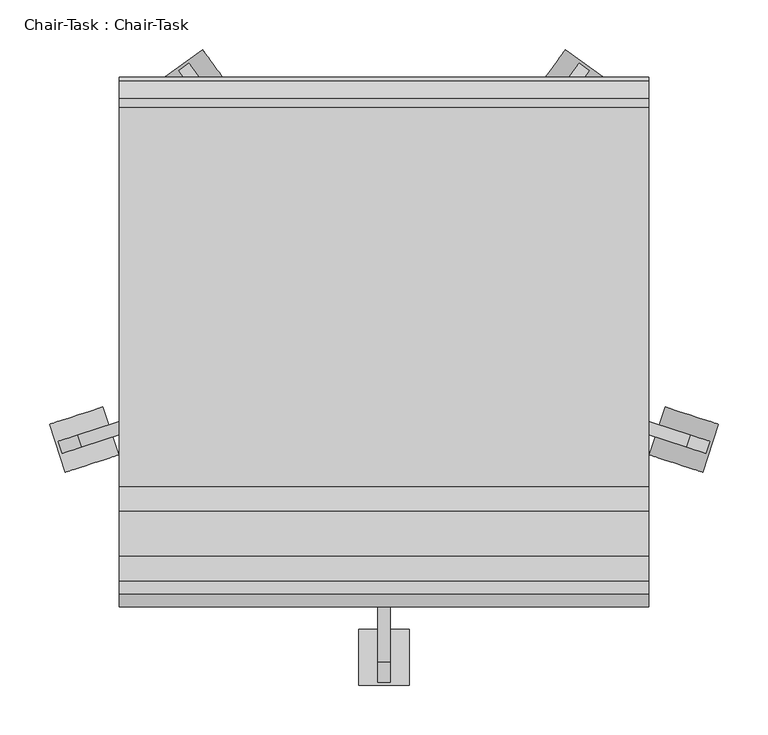
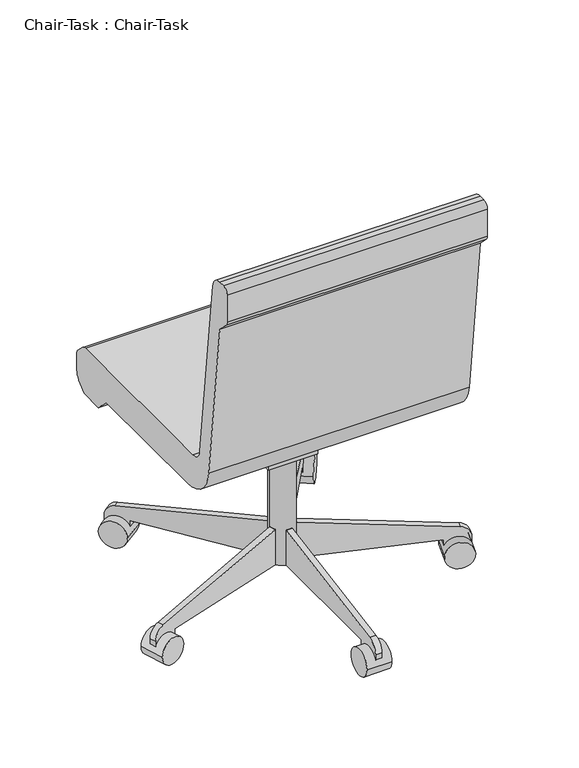
"""IFC4 building model written with IfcOpenShell, lengths in millimetres: furniture geometry, Chair-Task : Chair-Task."""

import ifcopenshell
import ifcopenshell.guid

model = None  # the IFC model being written
_history = None  # IfcOwnerHistory: only IFC2X3 demands one
_inside = {}  # id of a spatial element -> (the spatial element, [elements in it])
_under = {}  # id of a project, library or spatial element -> (it, [spatial elements below it])
_declared = {}  # id of a project -> (the project, [libraries it declares])
_typed = {}  # id of a type object -> (the type object, [elements of that type])
_made_of = {}  # id of a material, layer set ... -> (it, [elements and type objects made of it])


def new_model(schema):
    """Start an empty IFC model of exactly this schema.

    Asked for "IFC4X3", IfcOpenShell would pick the latest addendum, in which some entities
    have other attributes; the version numbers below select the first issue.
    IFC2X3 requires an IfcOwnerHistory on every rooted entity: one is made here for all.
    """
    global model, _history
    if schema == "IFC4X3":
        model = ifcopenshell.file(schema_version=(4, 3, 0, 0))
    else:
        model = ifcopenshell.file(schema=schema)
    _inside.clear()
    _under.clear()
    _declared.clear()
    _typed.clear()
    _made_of.clear()
    _history = None
    if model.schema == "IFC2X3":
        org = make("IfcOrganization", Name="unknown")
        user = make(
            "IfcPersonAndOrganization",
            ThePerson=make("IfcPerson", FamilyName="unknown"),
            TheOrganization=org,
        )
        app = make(
            "IfcApplication",
            ApplicationDeveloper=org,
            Version="unknown",
            ApplicationFullName="unknown",
            ApplicationIdentifier="unknown",
        )
        _history = make(
            "IfcOwnerHistory",
            OwningUser=user,
            OwningApplication=app,
            ChangeAction="ADDED",
            CreationDate=0,
        )
    return model


def make(cls, **values):
    """One entity of the class cls with the attributes given. An attribute that is None is left unset."""
    return model.create_entity(
        cls, **{name: value for name, value in values.items() if value is not None}
    )


def rooted(cls, **values):
    """An entity with a GlobalId (a new one), such as an element, a storey or a relation."""
    return make(cls, GlobalId=ifcopenshell.guid.new(), OwnerHistory=_history, **values)


def si_unit(unit_type, name, prefix=None):
    """IfcSIUnit, for example si_unit("LENGTHUNIT", "METRE", prefix="MILLI")."""
    return make("IfcSIUnit", UnitType=unit_type, Prefix=prefix, Name=name)


def assignment(units):
    """IfcUnitAssignment: the units of a project."""
    return None if units is None else make("IfcUnitAssignment", Units=units)


def point(xyz):
    """IfcCartesianPoint."""
    return None if xyz is None else make("IfcCartesianPoint", Coordinates=xyz)


def direction(xyz):
    """IfcDirection."""
    return None if xyz is None else make("IfcDirection", DirectionRatios=xyz)


def frame(location, z_axis=None, x_axis=None):
    """IfcAxis2Placement3D, a coordinate frame: its origin and axes. An axis left out is left unset."""
    return make(
        "IfcAxis2Placement3D",
        Location=point(location),
        Axis=direction(z_axis),
        RefDirection=direction(x_axis),
    )


def frame_2d(location, x_axis=None):
    """IfcAxis2Placement2D, a coordinate frame in the plane: its origin and x axis."""
    return make(
        "IfcAxis2Placement2D", Location=point(location), RefDirection=direction(x_axis)
    )


def origin():
    """The frame at (0, 0, 0) with its axes left unset."""
    return frame((0.0, 0.0, 0.0))


def place(relative_to, where):
    """IfcLocalPlacement: puts the frame where relative to a parent placement (None: the world)."""
    return make(
        "IfcLocalPlacement", PlacementRelTo=relative_to, RelativePlacement=where
    )


def context(
    kind, dimensions, precision=None, world=None, true_north=None, identifier=None
):
    """IfcGeometricRepresentationContext, for example the 3D "Model" context."""
    return make(
        "IfcGeometricRepresentationContext",
        ContextIdentifier=identifier,
        ContextType=kind,
        CoordinateSpaceDimension=dimensions,
        Precision=precision,
        WorldCoordinateSystem=world,
        TrueNorth=true_north,
    )


def project(units=None, contexts=None):
    """IfcProject with its units and contexts."""
    return rooted(
        "IfcProject",
        Name="project",
        RepresentationContexts=contexts,
        UnitsInContext=assignment(units),
    )


def spatial(cls, under=None, at=None, **own):
    """A site, building, storey or space (cls), placed at a placement, below another one or the project."""
    s = rooted(cls, ObjectPlacement=at, **own)
    if under is not None:
        _under.setdefault(under.id(), (under, []))[1].append(s)
    return s


def polyline(points):
    """IfcPolyline through the points."""
    return make("IfcPolyline", Points=[point(p) for p in points])


def circle_curve(where, radius):
    """IfcCircle in the frame where."""
    return make("IfcCircle", Position=where, Radius=radius)


def trimmed(basis, trim1, trim2, sense, master):
    """IfcTrimmedCurve: the piece of a basis curve between two trims."""
    return make(
        "IfcTrimmedCurve",
        BasisCurve=basis,
        Trim1=trim1,
        Trim2=trim2,
        SenseAgreement=sense,
        MasterRepresentation=master,
    )


def segment(curve, same_sense, transition):
    """IfcCompositeCurveSegment."""
    return make(
        "IfcCompositeCurveSegment",
        Transition=transition,
        SameSense=same_sense,
        ParentCurve=curve,
    )


def composite_curve(segments, self_intersect=None):
    """IfcCompositeCurve: segments joined end to end."""
    return make("IfcCompositeCurve", Segments=segments, SelfIntersect=self_intersect)


def outline(outer, holes=None, kind="AREA"):
    """IfcArbitraryClosedProfileDef: a profile drawn as a closed curve; with holes, ...WithVoids."""
    if holes is None:
        return make("IfcArbitraryClosedProfileDef", ProfileType=kind, OuterCurve=outer)
    return make(
        "IfcArbitraryProfileDefWithVoids",
        ProfileType=kind,
        OuterCurve=outer,
        InnerCurves=holes,
    )


def extrude(swept, where, along, depth):
    """IfcExtrudedAreaSolid: the profile swept, set in the frame where, extruded along a direction by depth."""
    return make(
        "IfcExtrudedAreaSolid",
        SweptArea=swept,
        Position=where,
        ExtrudedDirection=direction(along),
        Depth=depth,
    )


def shape(context_of_items, identifier, shape_type, items):
    """IfcShapeRepresentation: the items that make up one representation, for example the "Body"."""
    return make(
        "IfcShapeRepresentation",
        ContextOfItems=context_of_items,
        RepresentationIdentifier=identifier,
        RepresentationType=shape_type,
        Items=items,
    )


def source(mapping_origin, context_of_items, identifier, shape_type, items):
    """IfcRepresentationMap: a shape defined once, which mapped items show again and again."""
    return make(
        "IfcRepresentationMap",
        MappingOrigin=mapping_origin,
        MappedRepresentation=shape(context_of_items, identifier, shape_type, items),
    )


def transform(
    local_origin,
    x_axis=None,
    y_axis=None,
    z_axis=None,
    scale=None,
    scale2=None,
    scale3=None,
    uniform=True,
):
    """IfcCartesianTransformationOperator3D, or its non-uniform kind. x_axis, y_axis, z_axis: its Axis1, 2, 3."""
    if uniform:
        return make(
            "IfcCartesianTransformationOperator3D",
            Axis1=direction(x_axis),
            Axis2=direction(y_axis),
            LocalOrigin=point(local_origin),
            Scale=scale,
            Axis3=direction(z_axis),
        )
    return make(
        "IfcCartesianTransformationOperator3DnonUniform",
        Axis1=direction(x_axis),
        Axis2=direction(y_axis),
        LocalOrigin=point(local_origin),
        Scale=scale,
        Axis3=direction(z_axis),
        Scale2=scale2,
        Scale3=scale3,
    )


def mapped(mapping_source, mapping_target):
    """IfcMappedItem: shows the shape of a source again, moved by a transform."""
    return make(
        "IfcMappedItem", MappingSource=mapping_source, MappingTarget=mapping_target
    )


def made_of(thing, what):
    """Note that an element or type object is made of a material, layer set ...; save() writes the relation."""
    if what is not None:
        _made_of.setdefault(what.id(), (what, []))[1].append(thing)
    return thing


def element(
    cls,
    number,
    at=None,
    inside=None,
    cuts=None,
    type_object=None,
    material=None,
    context=None,
    identifier="Body",
    shape_type=None,
    held_by="IfcProductDefinitionShape",
    body=None,
    shapes=None,
    **own,
):
    """One element of the class cls, such as IfcWall. Its Tag is "e" and its number.

    at: its placement. inside: the storey or other place that contains it. cuts: it is an
    opening in that element (IfcRelVoidsElement). A single representation is given by context,
    identifier, shape_type and body (its items); several are given by shapes. held_by: the class
    of the entity that holds the representations. save() writes the other relations.
    """
    e = rooted(cls, Tag="e%d" % number, ObjectPlacement=at, **own)
    if body is not None:
        shapes = [shape(context, identifier, shape_type, body)]
    if shapes is not None:
        e.Representation = make(held_by, Representations=shapes)
    if inside is not None:
        _inside.setdefault(inside.id(), (inside, []))[1].append(e)
    if cuts is not None:
        rooted(
            "IfcRelVoidsElement", RelatingBuildingElement=cuts, RelatedOpeningElement=e
        )
    if type_object is not None:
        _typed.setdefault(type_object.id(), (type_object, []))[1].append(e)
    return made_of(e, material)


def aggregate(whole, parts):
    """IfcRelAggregates: a whole, such as a stair, and the parts it consists of."""
    return rooted("IfcRelAggregates", RelatingObject=whole, RelatedObjects=parts)


def save(model, path):
    """Write the relations noted so far, then the file.

    IfcRelAggregates (storeys below a building ...), IfcRelContainedInSpatialStructure (elements
    in a storey), IfcRelDefinesByType, IfcRelAssociatesMaterial and IfcRelDeclares: one each for
    every whole, place, type object, material and project.
    """
    for whole, parts in _under.values():
        aggregate(whole, parts)
    for where, things in _inside.values():
        rooted(
            "IfcRelContainedInSpatialStructure",
            RelatedElements=things,
            RelatingStructure=where,
        )
    for kind, things in _typed.values():
        rooted("IfcRelDefinesByType", RelatedObjects=things, RelatingType=kind)
    for what, things in _made_of.values():
        rooted("IfcRelAssociatesMaterial", RelatedObjects=things, RelatingMaterial=what)
    for by, libraries in _declared.values():
        rooted("IfcRelDeclares", RelatingContext=by, RelatedDefinitions=libraries)
    model.write(path)


def chair_task_chair_task_e9ee4668(model_context):
    return source(origin(), model_context, "Body", "SweptSolid", [
        extrude(outline(composite_curve([segment(trimmed(circle_curve(frame_2d((0.0, -28.2002728)), 28.2002727), [point((0.0, -56.4005455))], [point((0.0, 0.0))], False, "CARTESIAN"), True, "CONTINUOUS"), segment(trimmed(circle_curve(frame_2d((0.0, -28.2002728)), 28.2002727), [point((0.0, 0.0))], [point((0.0, -56.4005455))], False, "CARTESIAN"), True, "CONTINUOUS")], self_intersect=False)), frame((461.9222851, -112.0381931, 28.1835944), z_axis=(0.30901699437494234, 0.9510565162951552, 0.0), x_axis=(0.0, 0.0, 1.0)), (0.0, 0.0, 1.0), 50.8),
        extrude(outline(composite_curve([segment(polyline([(292.1, 0.0), (292.1, 25.4), (342.9, 25.4), (342.9, 1.096947)]), True, "CONTINUOUS"), segment(trimmed(circle_curve(frame_2d((317.5, 1.096947)), 25.4), [point((342.9, 1.096947))], [point((321.9106636, -23.9171699))], False, "CARTESIAN"), True, "CONTINUOUS"), segment(polyline([(321.9106636, -23.9171699), (25.4, -76.2), (0.0, -76.2), (0.0, 0.0), (292.1, 0.0)]), True, "CONTINUOUS")], self_intersect=False)), frame((139.0285618, 12.9066928, 53.5835944), z_axis=(0.30901699437494234, 0.9510565162951552, 0.0), x_axis=(0.9510565162951552, -0.30901699437494234, 0.0)), (0.0, 0.0, 1.0), 12.7),
        extrude(outline(composite_curve([segment(trimmed(circle_curve(frame_2d((0.0, -28.2002727)), 28.2002727), [point((0.0, -56.4005454))], [point((0.0, 0.0))], False, "CARTESIAN"), True, "CONTINUOUS"), segment(trimmed(circle_curve(frame_2d((0.0, -28.2002727)), 28.2002727), [point((0.0, 0.0))], [point((0.0, -56.4005454))], False, "CARTESIAN"), True, "CONTINUOUS")], self_intersect=False)), frame((364.7373733, 283.6935518, 28.1835944), z_axis=(-0.8090169943749497, 0.58778525229247, 0.0), x_axis=(0.0, 0.0, 1.0)), (0.0, 0.0, 1.0), 50.8),
        extrude(outline(composite_curve([segment(polyline([(292.1, 0.0), (292.1, 25.4), (342.9, 25.4), (342.9, 1.096947)]), True, "CONTINUOUS"), segment(trimmed(circle_curve(frame_2d((317.5, 1.096947)), 25.4), [point((342.9, 1.096947))], [point((321.9106637, -23.9171699))], False, "CARTESIAN"), True, "CONTINUOUS"), segment(polyline([(321.9106637, -23.9171699), (25.3999999, -76.2), (0.0, -76.2), (0.0, 0.0), (292.1, 0.0)]), True, "CONTINUOUS")], self_intersect=False)), frame((146.1280776, 15.2134653, 53.5835944), z_axis=(-0.8090169943749498, 0.58778525229247, 0.0), x_axis=(0.58778525229247, 0.8090169943749498, 0.0)), (0.0, 0.0, 1.0), 12.7),
        extrude(outline(composite_curve([segment(trimmed(circle_curve(frame_2d((0.0, -28.2002727)), 28.2002727), [point((0.0, -56.4005454))], [point((0.0, 0.0))], False, "CARTESIAN"), True, "CONTINUOUS"), segment(trimmed(circle_curve(frame_2d((0.0, -28.2002727)), 28.2002727), [point((0.0, 0.0))], [point((0.0, -56.4005454))], False, "CARTESIAN"), True, "CONTINUOUS")], self_intersect=False)), frame((-82.755734, 283.6935518, 28.1835944), z_axis=(0.8090169943749459, 0.5877852522924751, 0.0), x_axis=(0.0, 0.0, -1.0)), (0.0, 0.0, 1.0), 50.8),
        extrude(outline(composite_curve([segment(polyline([(-292.1, 0.0), (0.0, 0.0), (0.0, -76.2), (-25.4, -76.2), (-321.9106637, -23.9171699)]), True, "CONTINUOUS"), segment(trimmed(circle_curve(frame_2d((-317.5, 1.096947)), 25.4), [point((-321.9106637, -23.9171699))], [point((-342.9000001, 1.096947))], False, "CARTESIAN"), True, "CONTINUOUS"), segment(polyline([(-342.9000001, 1.096947), (-342.9000001, 25.4), (-292.1, 25.4), (-292.1, 0.0)]), True, "CONTINUOUS")], self_intersect=False)), frame((135.8535618, 15.2134653, 53.5835944), z_axis=(0.8090169943749459, 0.5877852522924752, 0.0), x_axis=(0.5877852522924752, -0.8090169943749459, 0.0)), (0.0, 0.0, 1.0), 12.7),
        extrude(outline(composite_curve([segment(trimmed(circle_curve(frame_2d((0.0, -28.2002727)), 28.2002727), [point((0.0, -56.4005454))], [point((0.0, 0.0))], False, "CARTESIAN"), True, "CONTINUOUS"), segment(trimmed(circle_curve(frame_2d((0.0, -28.2002727)), 28.2002727), [point((0.0, 0.0))], [point((0.0, -56.4005454))], False, "CARTESIAN"), True, "CONTINUOUS")], self_intersect=False)), frame((-179.9406457, -112.0381931, 28.1835944), z_axis=(-0.30901699437494856, 0.9510565162951532, 0.0), x_axis=(0.0, 0.0, -1.0)), (0.0, 0.0, 1.0), 50.8),
        extrude(outline(composite_curve([segment(polyline([(-292.1, 0.0), (0.0, 0.0), (0.0, -76.2), (-25.4, -76.2), (-321.9106637, -23.9171699)]), True, "CONTINUOUS"), segment(trimmed(circle_curve(frame_2d((-317.5, 1.096947)), 25.4), [point((-321.9106637, -23.9171699))], [point((-342.9000001, 1.096947))], False, "CARTESIAN"), True, "CONTINUOUS"), segment(polyline([(-342.9000001, 1.096947), (-342.9000001, 25.4), (-292.1, 25.4), (-292.1, 0.0)]), True, "CONTINUOUS")], self_intersect=False)), frame((142.9530776, 12.9066928, 53.5835944), z_axis=(-0.30901699437494856, 0.9510565162951532, 0.0), x_axis=(0.9510565162951532, 0.30901699437494856, 0.0)), (0.0, 0.0, 1.0), 12.7),
        extrude(outline(composite_curve([segment(trimmed(circle_curve(frame_2d((-298.5540984, 28.1835944)), 28.2002727), [point((-270.3538256, 28.1835944))], [point((-326.7543711, 28.1835944))], False, "CARTESIAN"), True, "CONTINUOUS"), segment(trimmed(circle_curve(frame_2d((-298.5540984, 28.1835944)), 28.2002727), [point((-326.7543711, 28.1835944))], [point((-270.3538256, 28.1835944))], False, "CARTESIAN"), True, "CONTINUOUS")], self_intersect=False)), frame((115.5908197, 0.0, 0.0), z_axis=(1.0, 0.0, 0.0), x_axis=(0.0, 1.0, 0.0)), (0.0, 0.0, 1.0), 50.8),
        extrude(outline(composite_curve([segment(polyline([(-273.1540984, 53.5835944), (-273.1540984, 28.1835944), (-323.9540984, 28.1835944), (-323.9540984, 52.4866474)]), True, "CONTINUOUS"), segment(trimmed(circle_curve(frame_2d((-298.5540984, 52.4866474)), 25.4), [point((-323.9540984, 52.4866474))], [point((-302.9647621, 77.5007643))], False, "CARTESIAN"), True, "CONTINUOUS"), segment(polyline([(-302.9647621, 77.5007643), (-6.4540984, 129.7835944), (18.9459016, 129.7835944), (18.9459016, 53.5835944), (-273.1540984, 53.5835944)]), True, "CONTINUOUS")], self_intersect=False)), frame((134.6408197, 0.0, 0.0), z_axis=(1.0, 0.0, 0.0), x_axis=(0.0, 1.0, 0.0)), (0.0, 0.0, 1.0), 12.7),
        extrude(outline(composite_curve([segment(trimmed(circle_curve(frame_2d((140.9908197, 18.9459016)), 25.4), [point((115.5908197, 18.9459016))], [point((166.3908197, 18.9459016))], False, "CARTESIAN"), True, "CONTINUOUS"), segment(trimmed(circle_curve(frame_2d((140.9908197, 18.9459016)), 25.4), [point((166.3908197, 18.9459016))], [point((115.5908197, 18.9459016))], False, "CARTESIAN"), True, "CONTINUOUS")], self_intersect=False)), frame((0.0, 0.0, 53.5835944), z_axis=(0.0, 0.0, 1.0), x_axis=(1.0, 0.0, 0.0)), (0.0, 0.0, 1.0), 330.5914056),
        extrude(outline(polyline([(69.7459016, 383.7835944), (69.7459016, 371.0835944), (18.9459016, 283.0954134), (-19.1540984, 283.0954134), (-19.1540984, 383.7835944), (69.7459016, 383.7835944)])), frame((90.1908197, 0.0, 0.0), z_axis=(1.0, 0.0, 0.0), x_axis=(0.0, 1.0, 0.0)), (0.0, 0.0, 1.0), 101.6),
        extrude(outline(composite_curve([segment(polyline([(-126.2050455, 457.2), (255.0102301, 457.2)]), True, "CONTINUOUS"), segment(trimmed(circle_curve(frame_2d((255.0102301, 444.5)), 12.7), [point((255.0102301, 457.2))], [point((263.9604301, 453.510212))], False, "CARTESIAN"), True, "CONTINUOUS"), segment(polyline([(263.9604301, 453.510212), (281.8961016, 435.6939999)]), True, "CONTINUOUS"), segment(trimmed(circle_curve(frame_2d((272.9459016, 426.6837879)), 12.7), [point((281.8961016, 435.6939999))], [point((285.6459016, 426.6837879))], False, "CARTESIAN"), True, "CONTINUOUS"), segment(polyline([(285.6459016, 426.6837879), (285.6459016, 391.6405184)]), True, "CONTINUOUS"), segment(trimmed(circle_curve(frame_2d((260.2459016, 391.6405184)), 25.4), [point((285.6459016, 391.6405184))], [point((278.2663256, 373.7401184))], False, "CARTESIAN"), True, "CONTINUOUS"), segment(polyline([(278.2663256, 373.7401184), (260.2470284, 355.6), (209.4470284, 355.6), (181.0744602, 383.7835944), (-107.1089978, 383.7835944)]), True, "CONTINUOUS"), segment(trimmed(circle_curve(frame_2d((-107.1089978, 459.9835944)), 76.2), [point((-107.1089978, 383.7835944))], [point((-182.7870738, 451.0802913))], False, "CARTESIAN"), True, "CONTINUOUS"), segment(polyline([(-182.7870738, 451.0802913), (-222.3540984, 787.4), (-244.0343545, 809.0802561)]), True, "CONTINUOUS"), segment(trimmed(circle_curve(frame_2d((-235.0540984, 818.0605122)), 12.7), [point((-244.0343545, 809.0802561))], [point((-247.7540984, 818.0605122))], False, "CARTESIAN"), True, "CONTINUOUS"), segment(polyline([(-247.7540984, 818.0605122), (-247.7540984, 876.3)]), True, "CONTINUOUS"), segment(trimmed(circle_curve(frame_2d((-235.0540984, 876.3)), 12.7), [point((-247.7540984, 876.3))], [point((-235.0540984, 889.0))], False, "CARTESIAN"), True, "CONTINUOUS"), segment(polyline([(-235.0540984, 889.0), (-222.1789239, 889.0)]), True, "CONTINUOUS"), segment(trimmed(circle_curve(frame_2d((-222.1789239, 863.6)), 25.4), [point((-222.1789239, 889.0))], [point((-196.9528985, 866.5677677))], False, "CARTESIAN"), True, "CONTINUOUS"), segment(polyline([(-196.9528985, 866.5677677), (-151.4310708, 479.6322323)]), True, "CONTINUOUS"), segment(trimmed(circle_curve(frame_2d((-126.2050455, 482.6)), 25.4), [point((-151.4310708, 479.6322323))], [point((-126.2050455, 457.2))], True, "CARTESIAN"), True, "CONTINUOUS")], self_intersect=False)), frame((-125.7091803, 0.0, 0.0), z_axis=(1.0, 0.0, 0.0), x_axis=(0.0, 1.0, 0.0)), (0.0, 0.0, 1.0), 533.4),
    ])


if __name__ == "__main__":
    model = new_model("IFC4")
    model_context = context("Model", 3, world=origin())
    ifc_project = project(units=[si_unit("LENGTHUNIT", "METRE", prefix="MILLI")], contexts=[model_context])
    site = spatial("IfcSite", under=ifc_project)
    building = spatial("IfcBuilding", under=site)
    placement = place(None, origin())
    chair_task_chair_task_shape = chair_task_chair_task_e9ee4668(model_context)
    element("IfcFurniture", 1, ObjectType="Chair-Task : Chair-Task", at=placement, inside=building, context=model_context, shape_type="MappedRepresentation", body=[
        mapped(chair_task_chair_task_shape, transform((0.0, 0.0, 0.0), x_axis=(1.0, 0.0, 0.0), y_axis=(0.0, 1.0, 0.0), z_axis=(0.0, 0.0, 1.0))),
    ])
    save(model, "model.ifc")

# Revit data of these elements
# Type "Chair-Task : Chair-Task"
#   Model = "CHTSK-895"
#   Manufacturer = "Furniture Concepts"
#   Type Mark = "CH-4"
#   Assembly Code = "E2020200"
#   Cost = 895
#   Base Material = Plastic, Opaque Black
#   Caster Material = Plastic, Opaque Black
#   Seat/Back Material = Leather - Matte (Tan)
#   Default Elevation = 0
# Element 1 (IfcFurniture, "Chair-Task : Chair-Task")
#   Materials on its faces: "Plastic, Opaque Black", "Leather - Matte (Tan)"
# Materials
#   "Plastic, Opaque Black": class "Plastic", colour RGB 0 0 0, transparency 0, Description = "Plastic, generic, opaque black", Cost = 0
#   "Leather - Matte (Tan)": class "Generic", colour RGB 162 130 69, transparency 0, Cost = 0
